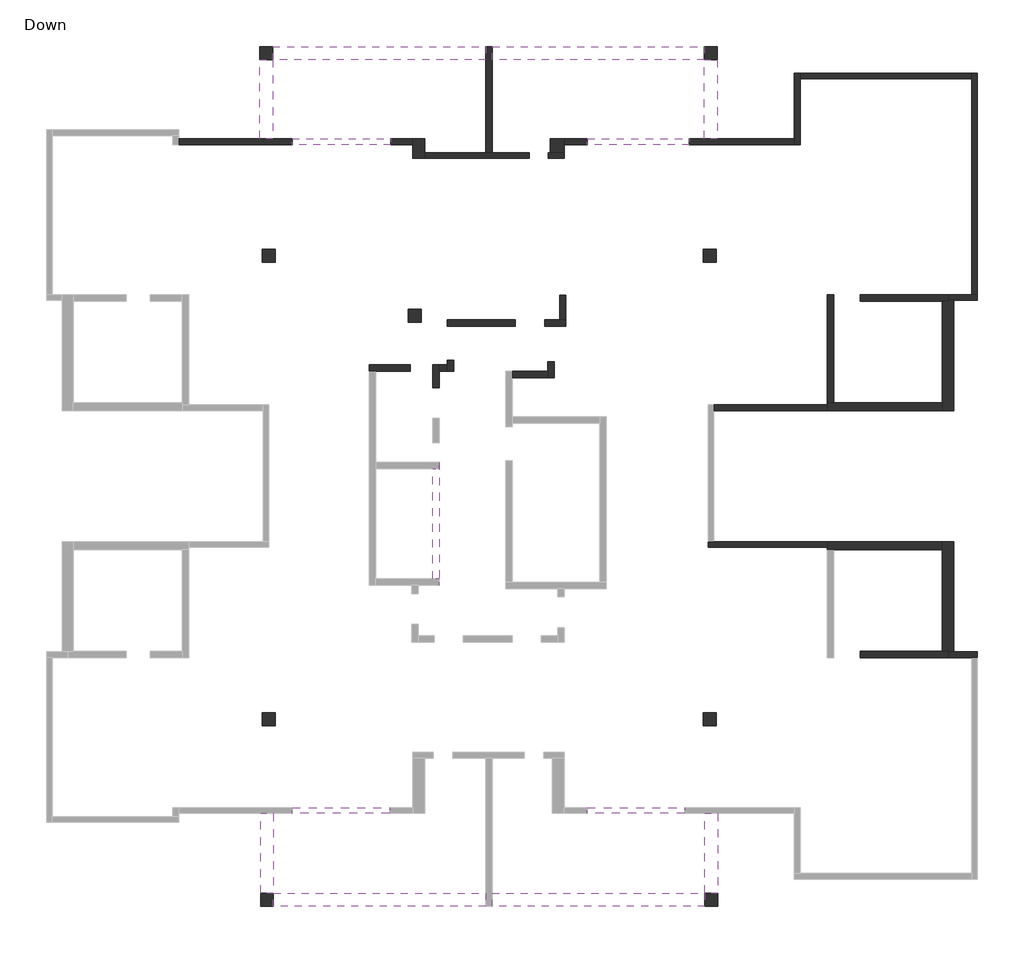
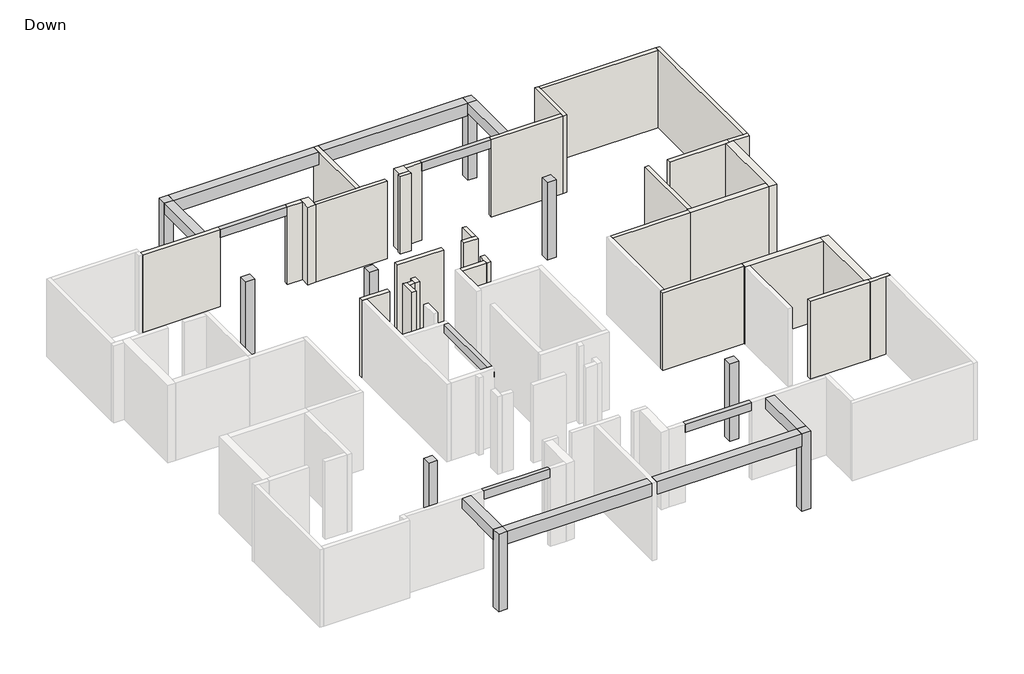
# One storey, part 2 of 2: 32 walls, 13 beams, 9 columns.
# Revit data of these elements (continued)
# Element 27 (IfcWall, "18") (continued)
#   SOFiSTiK_AMG_Scheduled = yes
#   SOFiSTiK_AMG_Adjusted = yes
#   Phase Created = New Construction
#   Base Constraint = Down
#   Top Constraint = Typical Floor
#   Materials on its faces: "Concrete"
# Element 28 (IfcWall, "18")
#   Comments = ""
#   Mark = "W28"
#   SOFiSTiK_EdgeZones = "W28"
#   SOFiSTiK_AMG_Comments = ""
#   Top Offset = 0 cm
#   Base Offset = 0 cm
#   wall height = 370 cm
#   SOFiSTiK_AMG_Scheduled = yes
#   SOFiSTiK_AMG_Adjusted = yes
#   Phase Created = New Construction
#   Base Constraint = Down
#   Top Constraint = Typical Floor
#   Materials on its faces: "Concrete"
# Element 29 (IfcWall, "18")
#   Comments = ""
#   Mark = "W29"
#   SOFiSTiK_EdgeZones = "W29"
#   SOFiSTiK_AMG_Comments = ""
#   Top Offset = 0 cm
#   Base Offset = 0 cm
#   wall height = 370 cm
#   SOFiSTiK_AMG_Scheduled = yes
#   SOFiSTiK_AMG_Adjusted = yes
#   Phase Created = New Construction
#   Base Constraint = Down
#   Top Constraint = Typical Floor
#   Materials on its faces: "Concrete"
# Element 30 (IfcWall, "18")
#   Comments = ""
#   Mark = "W30"
#   SOFiSTiK_EdgeZones = "W30"
#   SOFiSTiK_AMG_Comments = ""
#   Top Offset = 0 cm
#   Base Offset = 0 cm
#   wall height = 370 cm
#   SOFiSTiK_AMG_Scheduled = yes
#   SOFiSTiK_AMG_Adjusted = yes
#   Phase Created = New Construction
#   Base Constraint = Down
#   Top Constraint = Typical Floor
#   Materials on its faces: "Concrete"
# Element 31 (IfcWall, "18")
#   Comments = ""
#   Mark = "W31"
#   SOFiSTiK_EdgeZones = "W31"
#   SOFiSTiK_AMG_Comments = ""
#   Top Offset = 0 cm
#   Base Offset = 0 cm
#   wall height = 370 cm
#   SOFiSTiK_AMG_Scheduled = yes
#   SOFiSTiK_AMG_Adjusted = yes
#   Phase Created = New Construction
#   Base Constraint = Down
#   Top Constraint = Typical Floor
#   Materials on its faces: "Concrete"
# Element 32 (IfcWall, "18")
#   Comments = ""
#   Mark = "W32"
#   SOFiSTiK_EdgeZones = "W32"
#   SOFiSTiK_AMG_Comments = ""
#   Top Offset = 0 cm
#   Base Offset = 0 cm
#   wall height = 370 cm
#   SOFiSTiK_AMG_Scheduled = yes
#   SOFiSTiK_AMG_Adjusted = yes
#   Phase Created = New Construction
#   Base Constraint = Down
#   Top Constraint = Typical Floor
#   Materials on its faces: "Concrete"
# Element 33 (IfcWall, "18")
#   Comments = ""
#   Mark = "W33"
#   SOFiSTiK_EdgeZones = "W33"
#   SOFiSTiK_AMG_Comments = ""
#   Top Offset = 0 cm
#   Base Offset = 0 cm
#   wall height = 370 cm
#   SOFiSTiK_AMG_Scheduled = yes
#   SOFiSTiK_AMG_Adjusted = yes
#   Phase Created = New Construction
#   Base Constraint = Down
#   Top Constraint = Typical Floor
#   Materials on its faces: "Concrete"
# Element 34 (IfcWall, "18")
#   Comments = ""
#   Mark = "W34"
#   SOFiSTiK_EdgeZones = "W35"
#   SOFiSTiK_AMG_Comments = ""
#   Top Offset = 0 cm
#   Base Offset = 0 cm
#   wall height = 370 cm
#   SOFiSTiK_AMG_Scheduled = yes
#   SOFiSTiK_AMG_Adjusted = yes
#   Phase Created = New Construction
#   Base Constraint = Down
#   Top Constraint = Typical Floor
#   Materials on its faces: "Concrete"
# Element 35 (IfcWall, "18")
#   Comments = ""
#   Mark = "W35"
#   SOFiSTiK_EdgeZones = "W36"
#   SOFiSTiK_AMG_Comments = ""
#   Top Offset = 0 cm
#   Base Offset = 0 cm
#   wall height = 370 cm
#   SOFiSTiK_AMG_Scheduled = yes
#   SOFiSTiK_AMG_Adjusted = yes
#   Phase Created = New Construction
#   Base Constraint = Down
#   Top Constraint = Typical Floor
#   Materials on its faces: "Concrete"
# Element 36 (IfcWall, "18")
#   Comments = ""
#   Mark = "W36"
#   SOFiSTiK_EdgeZones = "W38"
#   SOFiSTiK_AMG_Comments = ""
#   Top Offset = 0 cm
#   Base Offset = 0 cm
#   wall height = 370 cm
#   SOFiSTiK_AMG_Scheduled = yes
#   SOFiSTiK_AMG_Adjusted = yes
#   Phase Created = New Construction
#   Base Constraint = Down
#   Top Constraint = Typical Floor
#   Materials on its faces: "Concrete"
# Element 37 (IfcWall, "20")
#   Comments = ""
#   Mark = "W44"
#   SOFiSTiK_EdgeZones = "W46"
#   SOFiSTiK_AMG_Comments = ""
#   Top Offset = 0 cm
#   Base Offset = 0 cm
#   wall height = 370 cm
#   SOFiSTiK_AMG_Scheduled = yes
#   SOFiSTiK_AMG_Adjusted = yes
#   Phase Created = New Construction
#   Base Constraint = Down
#   Top Constraint = Typical Floor
#   Materials on its faces: "Concrete"
# Element 38 (IfcWall, "20")
#   Comments = ""
#   Mark = "W49"
#   SOFiSTiK_EdgeZones = "W51"
#   SOFiSTiK_AMG_Comments = ""
#   Top Offset = 0 cm
#   Base Offset = 0 cm
#   wall height = 370 cm
#   SOFiSTiK_AMG_Scheduled = yes
#   SOFiSTiK_AMG_Adjusted = yes
#   Phase Created = New Construction
#   Base Constraint = Down
#   Top Constraint = Typical Floor
#   Materials on its faces: "Concrete"
# Element 39 (IfcWall, "20")
#   Comments = ""
#   Mark = "W50"
#   SOFiSTiK_EdgeZones = "W52"
#   SOFiSTiK_AMG_Comments = ""
#   Top Offset = 0 cm
#   Base Offset = 0 cm
#   wall height = 370 cm
#   SOFiSTiK_AMG_Scheduled = yes
#   SOFiSTiK_AMG_Adjusted = yes
#   Phase Created = New Construction
#   Base Constraint = Down
#   Top Constraint = Typical Floor
#   Materials on its faces: "Concrete"
# Element 40 (IfcWall, "20")
#   Comments = ""
#   Mark = "W51"
#   SOFiSTiK_EdgeZones = "W53"
#   SOFiSTiK_AMG_Comments = ""
#   Top Offset = 0 cm
#   Base Offset = 0 cm
#   wall height = 370 cm
#   SOFiSTiK_AMG_Scheduled = yes
#   SOFiSTiK_AMG_Adjusted = yes
#   Phase Created = New Construction
#   Base Constraint = Down
#   Top Constraint = Typical Floor
#   Materials on its faces: "Concrete"
# Element 41 (IfcWall, "20")
#   Comments = ""
#   Mark = "W64"
#   SOFiSTiK_EdgeZones = "W66"
#   SOFiSTiK_AMG_Comments = ""
#   Top Offset = 0 cm
#   Base Offset = 0 cm
#   wall height = 370 cm
#   SOFiSTiK_AMG_Scheduled = yes
#   SOFiSTiK_AMG_Adjusted = yes
#   Phase Created = New Construction
#   Base Constraint = Down
#   Top Constraint = Typical Floor
#   Materials on its faces: "Concrete"
# Element 42 (IfcWall, "20")
#   Comments = ""
#   Mark = "W65"
#   SOFiSTiK_EdgeZones = "W67"
#   SOFiSTiK_AMG_Comments = ""
#   Top Offset = 0 cm
#   Base Offset = 0 cm
#   wall height = 370 cm
#   SOFiSTiK_AMG_Scheduled = yes
#   SOFiSTiK_AMG_Adjusted = yes
#   Phase Created = New Construction
#   Base Constraint = Down
#   Top Constraint = Typical Floor
#   Materials on its faces: "Concrete"
# Element 43 (IfcWall, "20")
#   Comments = ""
#   Mark = "W66"
#   SOFiSTiK_EdgeZones = "W68"
#   SOFiSTiK_AMG_Comments = ""
#   Top Offset = 0 cm
#   Base Offset = 0 cm
#   wall height = 370 cm
#   SOFiSTiK_AMG_Scheduled = yes
#   SOFiSTiK_AMG_Adjusted = yes
#   Phase Created = New Construction
#   Base Constraint = Down
#   Top Constraint = Typical Floor
#   Materials on its faces: "Concrete"
# Element 44 (IfcWall, "20")
#   Comments = ""
#   Mark = "W67"
#   SOFiSTiK_EdgeZones = "W69"
#   SOFiSTiK_AMG_Comments = ""
#   Top Offset = 0 cm
#   Base Offset = 0 cm
#   wall height = 370 cm
#   SOFiSTiK_AMG_Scheduled = yes
#   SOFiSTiK_AMG_Adjusted = yes
#   Phase Created = New Construction
#   Base Constraint = Down
#   Top Constraint = Typical Floor
#   Materials on its faces: "Concrete"
# Element 45 (IfcWall, "20")
#   Comments = ""
#   Mark = "W68"
#   SOFiSTiK_EdgeZones = "W70"
#   SOFiSTiK_AMG_Comments = ""
#   Top Offset = 0 cm
#   Base Offset = 0 cm
#   wall height = 370 cm
#   SOFiSTiK_AMG_Scheduled = yes
#   SOFiSTiK_AMG_Adjusted = yes
#   Phase Created = New Construction
#   Base Constraint = Down
#   Top Constraint = Typical Floor
#   Materials on its faces: "Concrete"
# Element 46 (IfcWall, "20")
#   Comments = ""
#   Mark = "W69"
#   SOFiSTiK_EdgeZones = "W71"
#   SOFiSTiK_AMG_Comments = ""
#   Top Offset = 0 cm
#   Base Offset = 0 cm
#   wall height = 370 cm
#   SOFiSTiK_AMG_Scheduled = yes
#   SOFiSTiK_AMG_Adjusted = yes
#   Phase Created = New Construction
#   Base Constraint = Down
#   Top Constraint = Typical Floor
#   Materials on its faces: "Concrete"
# Element 47 (IfcWall, "20")
#   Comments = ""
#   Mark = "W70"
#   SOFiSTiK_EdgeZones = "W72"
#   SOFiSTiK_AMG_Comments = ""
#   Top Offset = 0 cm
#   Base Offset = 0 cm
#   wall height = 370 cm
#   SOFiSTiK_AMG_Scheduled = yes
#   SOFiSTiK_AMG_Adjusted = yes
#   Phase Created = New Construction
#   Base Constraint = Down
#   Top Constraint = Typical Floor
#   Materials on its faces: "Concrete"
# Element 48 (IfcWall, "20")
#   Comments = ""
#   Mark = "W72"
#   SOFiSTiK_EdgeZones = "W74"
#   SOFiSTiK_AMG_Comments = ""
#   Top Offset = 0 cm
#   Base Offset = 0 cm
#   wall height = 370 cm
#   SOFiSTiK_AMG_Scheduled = yes
#   SOFiSTiK_AMG_Adjusted = yes
#   Phase Created = New Construction
#   Base Constraint = Down
#   Top Constraint = Typical Floor
#   Materials on its faces: "Concrete"
# Element 49 (IfcWall, "25")
#   Comments = ""
#   Mark = "W81"
#   SOFiSTiK_EdgeZones = "W83"
#   SOFiSTiK_AMG_Comments = ""
#   Top Offset = 0 cm
#   Base Offset = 0 cm
#   wall height = 370 cm
#   SOFiSTiK_AMG_Scheduled = yes
#   SOFiSTiK_AMG_Adjusted = yes
#   Phase Created = New Construction
#   Base Constraint = Down
#   Top Constraint = Typical Floor
#   Materials on its faces: "Concrete"
# Element 50 (IfcWall, "25")
#   Comments = ""
#   Mark = "W83"
#   SOFiSTiK_EdgeZones = "W85"
#   SOFiSTiK_AMG_Comments = ""
#   Top Offset = 0 cm
#   Base Offset = 0 cm
#   wall height = 370 cm
#   SOFiSTiK_AMG_Scheduled = yes
#   SOFiSTiK_AMG_Adjusted = yes
#   Phase Created = New Construction
#   Base Constraint = Down
#   Top Constraint = Typical Floor
#   Materials on its faces: "Concrete"
# Element 51 (IfcWall, "35")
#   Comments = ""
#   Mark = "W77"
#   SOFiSTiK_EdgeZones = "W79"
#   SOFiSTiK_AMG_Comments = ""
#   Top Offset = 0 cm
#   Base Offset = 0 cm
#   wall height = 370 cm
#   SOFiSTiK_AMG_Scheduled = yes
#   SOFiSTiK_AMG_Adjusted = yes
#   Phase Created = New Construction
#   Base Constraint = Down
#   Top Constraint = Typical Floor
#   Materials on its faces: "Concrete"
# Element 52 (IfcWall, "35")
#   Comments = ""
#   Mark = "W79"
#   SOFiSTiK_EdgeZones = "W81"
#   SOFiSTiK_AMG_Comments = ""
#   Top Offset = 0 cm
#   Base Offset = 0 cm
#   wall height = 370 cm
#   SOFiSTiK_AMG_Scheduled = yes
#   SOFiSTiK_AMG_Adjusted = yes
#   Phase Created = New Construction
#   Base Constraint = Down
#   Top Constraint = Typical Floor
#   Materials on its faces: "Concrete"
# Element 53 (IfcWall, "36")
#   Comments = ""
#   Mark = "W39"
#   SOFiSTiK_EdgeZones = "W41"
#   SOFiSTiK_AMG_Comments = ""
#   Top Offset = 0 cm
#   Base Offset = 0 cm
#   wall height = 370 cm
#   SOFiSTiK_AMG_Scheduled = yes
#   SOFiSTiK_AMG_Adjusted = yes
#   Phase Created = New Construction
#   Base Constraint = Down
#   Top Constraint = Typical Floor
#   Materials on its faces: "Concrete"
# Element 54 (IfcWall, "43")
#   Comments = ""
#   Mark = "W84"
#   SOFiSTiK_AMG_Comments = ""
#   Top Offset = 0 cm
#   Base Offset = 0 cm
#   wall height = 370 cm
#   SOFiSTiK_AMG_Scheduled = yes
#   SOFiSTiK_AMG_Adjusted = yes
#   Phase Created = New Construction
#   Base Constraint = Down
#   Top Constraint = Typical Floor
#   Materials on its faces: "Concrete"
# Materials
#   "Concrete": class "Concrete", colour RGB 192 192 192, transparency 0, Keynote = "01000", Description = "Cast-in-place concrete", Cost = 0
